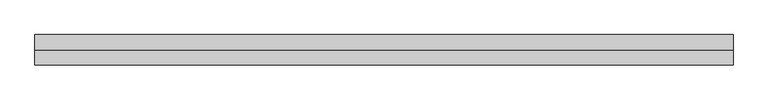
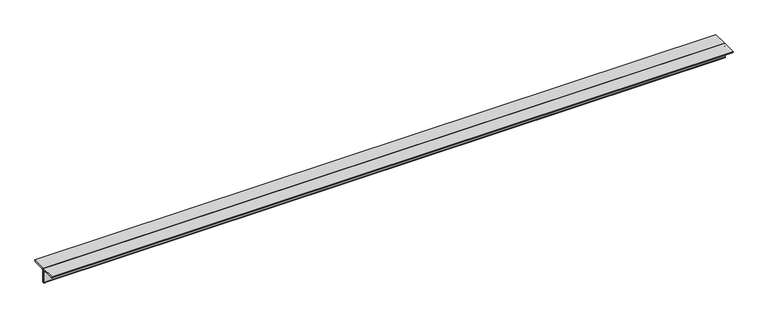
"""IFC4 building model written with IfcOpenShell, lengths in millimetres: member geometry, 0123_Steel Framing_2Ls-KSD3502 : H_SB_AR_S03_2Ls-130x130x12_HBR1."""

import ifcopenshell
import ifcopenshell.guid

model = None  # the IFC model being written
_history = None  # IfcOwnerHistory: only IFC2X3 demands one
_inside = {}  # id of a spatial element -> (the spatial element, [elements in it])
_under = {}  # id of a project, library or spatial element -> (it, [spatial elements below it])
_declared = {}  # id of a project -> (the project, [libraries it declares])
_typed = {}  # id of a type object -> (the type object, [elements of that type])
_made_of = {}  # id of a material, layer set ... -> (it, [elements and type objects made of it])


def new_model(schema):
    """Start an empty IFC model of exactly this schema.

    Asked for "IFC4X3", IfcOpenShell would pick the latest addendum, in which some entities
    have other attributes; the version numbers below select the first issue.
    IFC2X3 requires an IfcOwnerHistory on every rooted entity: one is made here for all.
    """
    global model, _history
    if schema == "IFC4X3":
        model = ifcopenshell.file(schema_version=(4, 3, 0, 0))
    else:
        model = ifcopenshell.file(schema=schema)
    _inside.clear()
    _under.clear()
    _declared.clear()
    _typed.clear()
    _made_of.clear()
    _history = None
    if model.schema == "IFC2X3":
        org = make("IfcOrganization", Name="unknown")
        user = make(
            "IfcPersonAndOrganization",
            ThePerson=make("IfcPerson", FamilyName="unknown"),
            TheOrganization=org,
        )
        app = make(
            "IfcApplication",
            ApplicationDeveloper=org,
            Version="unknown",
            ApplicationFullName="unknown",
            ApplicationIdentifier="unknown",
        )
        _history = make(
            "IfcOwnerHistory",
            OwningUser=user,
            OwningApplication=app,
            ChangeAction="ADDED",
            CreationDate=0,
        )
    return model


def make(cls, **values):
    """One entity of the class cls with the attributes given. An attribute that is None is left unset."""
    return model.create_entity(
        cls, **{name: value for name, value in values.items() if value is not None}
    )


def rooted(cls, **values):
    """An entity with a GlobalId (a new one), such as an element, a storey or a relation."""
    return make(cls, GlobalId=ifcopenshell.guid.new(), OwnerHistory=_history, **values)


def si_unit(unit_type, name, prefix=None):
    """IfcSIUnit, for example si_unit("LENGTHUNIT", "METRE", prefix="MILLI")."""
    return make("IfcSIUnit", UnitType=unit_type, Prefix=prefix, Name=name)


def assignment(units):
    """IfcUnitAssignment: the units of a project."""
    return None if units is None else make("IfcUnitAssignment", Units=units)


def point(xyz):
    """IfcCartesianPoint."""
    return None if xyz is None else make("IfcCartesianPoint", Coordinates=xyz)


def direction(xyz):
    """IfcDirection."""
    return None if xyz is None else make("IfcDirection", DirectionRatios=xyz)


def frame(location, z_axis=None, x_axis=None):
    """IfcAxis2Placement3D, a coordinate frame: its origin and axes. An axis left out is left unset."""
    return make(
        "IfcAxis2Placement3D",
        Location=point(location),
        Axis=direction(z_axis),
        RefDirection=direction(x_axis),
    )


def frame_2d(location, x_axis=None):
    """IfcAxis2Placement2D, a coordinate frame in the plane: its origin and x axis."""
    return make(
        "IfcAxis2Placement2D", Location=point(location), RefDirection=direction(x_axis)
    )


def origin():
    """The frame at (0, 0, 0) with its axes left unset."""
    return frame((0.0, 0.0, 0.0))


def place(relative_to, where):
    """IfcLocalPlacement: puts the frame where relative to a parent placement (None: the world)."""
    return make(
        "IfcLocalPlacement", PlacementRelTo=relative_to, RelativePlacement=where
    )


def context(
    kind, dimensions, precision=None, world=None, true_north=None, identifier=None
):
    """IfcGeometricRepresentationContext, for example the 3D "Model" context."""
    return make(
        "IfcGeometricRepresentationContext",
        ContextIdentifier=identifier,
        ContextType=kind,
        CoordinateSpaceDimension=dimensions,
        Precision=precision,
        WorldCoordinateSystem=world,
        TrueNorth=true_north,
    )


def project(units=None, contexts=None):
    """IfcProject with its units and contexts."""
    return rooted(
        "IfcProject",
        Name="project",
        RepresentationContexts=contexts,
        UnitsInContext=assignment(units),
    )


def spatial(cls, under=None, at=None, **own):
    """A site, building, storey or space (cls), placed at a placement, below another one or the project."""
    s = rooted(cls, ObjectPlacement=at, **own)
    if under is not None:
        _under.setdefault(under.id(), (under, []))[1].append(s)
    return s


def polyline(points):
    """IfcPolyline through the points."""
    return make("IfcPolyline", Points=[point(p) for p in points])


def circle_curve(where, radius):
    """IfcCircle in the frame where."""
    return make("IfcCircle", Position=where, Radius=radius)


def trimmed(basis, trim1, trim2, sense, master):
    """IfcTrimmedCurve: the piece of a basis curve between two trims."""
    return make(
        "IfcTrimmedCurve",
        BasisCurve=basis,
        Trim1=trim1,
        Trim2=trim2,
        SenseAgreement=sense,
        MasterRepresentation=master,
    )


def segment(curve, same_sense, transition):
    """IfcCompositeCurveSegment."""
    return make(
        "IfcCompositeCurveSegment",
        Transition=transition,
        SameSense=same_sense,
        ParentCurve=curve,
    )


def composite_curve(segments, self_intersect=None):
    """IfcCompositeCurve: segments joined end to end."""
    return make("IfcCompositeCurve", Segments=segments, SelfIntersect=self_intersect)


def outline(outer, holes=None, kind="AREA"):
    """IfcArbitraryClosedProfileDef: a profile drawn as a closed curve; with holes, ...WithVoids."""
    if holes is None:
        return make("IfcArbitraryClosedProfileDef", ProfileType=kind, OuterCurve=outer)
    return make(
        "IfcArbitraryProfileDefWithVoids",
        ProfileType=kind,
        OuterCurve=outer,
        InnerCurves=holes,
    )


def extrude(swept, where, along, depth):
    """IfcExtrudedAreaSolid: the profile swept, set in the frame where, extruded along a direction by depth."""
    return make(
        "IfcExtrudedAreaSolid",
        SweptArea=swept,
        Position=where,
        ExtrudedDirection=direction(along),
        Depth=depth,
    )


def shape(context_of_items, identifier, shape_type, items):
    """IfcShapeRepresentation: the items that make up one representation, for example the "Body"."""
    return make(
        "IfcShapeRepresentation",
        ContextOfItems=context_of_items,
        RepresentationIdentifier=identifier,
        RepresentationType=shape_type,
        Items=items,
    )


def source(mapping_origin, context_of_items, identifier, shape_type, items):
    """IfcRepresentationMap: a shape defined once, which mapped items show again and again."""
    return make(
        "IfcRepresentationMap",
        MappingOrigin=mapping_origin,
        MappedRepresentation=shape(context_of_items, identifier, shape_type, items),
    )


def transform(
    local_origin,
    x_axis=None,
    y_axis=None,
    z_axis=None,
    scale=None,
    scale2=None,
    scale3=None,
    uniform=True,
):
    """IfcCartesianTransformationOperator3D, or its non-uniform kind. x_axis, y_axis, z_axis: its Axis1, 2, 3."""
    if uniform:
        return make(
            "IfcCartesianTransformationOperator3D",
            Axis1=direction(x_axis),
            Axis2=direction(y_axis),
            LocalOrigin=point(local_origin),
            Scale=scale,
            Axis3=direction(z_axis),
        )
    return make(
        "IfcCartesianTransformationOperator3DnonUniform",
        Axis1=direction(x_axis),
        Axis2=direction(y_axis),
        LocalOrigin=point(local_origin),
        Scale=scale,
        Axis3=direction(z_axis),
        Scale2=scale2,
        Scale3=scale3,
    )


def mapped(mapping_source, mapping_target):
    """IfcMappedItem: shows the shape of a source again, moved by a transform."""
    return make(
        "IfcMappedItem", MappingSource=mapping_source, MappingTarget=mapping_target
    )


def made_of(thing, what):
    """Note that an element or type object is made of a material, layer set ...; save() writes the relation."""
    if what is not None:
        _made_of.setdefault(what.id(), (what, []))[1].append(thing)
    return thing


def element(
    cls,
    number,
    at=None,
    inside=None,
    cuts=None,
    type_object=None,
    material=None,
    context=None,
    identifier="Body",
    shape_type=None,
    held_by="IfcProductDefinitionShape",
    body=None,
    shapes=None,
    **own,
):
    """One element of the class cls, such as IfcWall. Its Tag is "e" and its number.

    at: its placement. inside: the storey or other place that contains it. cuts: it is an
    opening in that element (IfcRelVoidsElement). A single representation is given by context,
    identifier, shape_type and body (its items); several are given by shapes. held_by: the class
    of the entity that holds the representations. save() writes the other relations.
    """
    e = rooted(cls, Tag="e%d" % number, ObjectPlacement=at, **own)
    if body is not None:
        shapes = [shape(context, identifier, shape_type, body)]
    if shapes is not None:
        e.Representation = make(held_by, Representations=shapes)
    if inside is not None:
        _inside.setdefault(inside.id(), (inside, []))[1].append(e)
    if cuts is not None:
        rooted(
            "IfcRelVoidsElement", RelatingBuildingElement=cuts, RelatedOpeningElement=e
        )
    if type_object is not None:
        _typed.setdefault(type_object.id(), (type_object, []))[1].append(e)
    return made_of(e, material)


def aggregate(whole, parts):
    """IfcRelAggregates: a whole, such as a stair, and the parts it consists of."""
    return rooted("IfcRelAggregates", RelatingObject=whole, RelatedObjects=parts)


def save(model, path):
    """Write the relations noted so far, then the file.

    IfcRelAggregates (storeys below a building ...), IfcRelContainedInSpatialStructure (elements
    in a storey), IfcRelDefinesByType, IfcRelAssociatesMaterial and IfcRelDeclares: one each for
    every whole, place, type object, material and project.
    """
    for whole, parts in _under.values():
        aggregate(whole, parts)
    for where, things in _inside.values():
        rooted(
            "IfcRelContainedInSpatialStructure",
            RelatedElements=things,
            RelatingStructure=where,
        )
    for kind, things in _typed.values():
        rooted("IfcRelDefinesByType", RelatedObjects=things, RelatingType=kind)
    for what, things in _made_of.values():
        rooted("IfcRelAssociatesMaterial", RelatedObjects=things, RelatingMaterial=what)
    for by, libraries in _declared.values():
        rooted("IfcRelDeclares", RelatingContext=by, RelatedDefinitions=libraries)
    model.write(path)


def member_93b6b39c(model_context):
    return source(origin(), model_context, "Body", "SweptSolid", [
        extrude(outline(composite_curve([segment(polyline([(0.0, 36.4), (130.0, 36.4)]), True, "CONTINUOUS"), segment(trimmed(circle_curve(frame_2d((118.0, 36.4)), 12.0), [point((130.0, 36.4))], [point((118.0, 24.4))], False, "CARTESIAN"), True, "CONTINUOUS"), segment(polyline([(118.0, 24.4), (24.0, 24.4)]), True, "CONTINUOUS"), segment(trimmed(circle_curve(frame_2d((24.0, 12.4)), 12.0), [point((24.0, 24.4))], [point((12.0, 12.4))], True, "CARTESIAN"), True, "CONTINUOUS"), segment(polyline([(12.0, 12.4), (12.0, -81.6)]), True, "CONTINUOUS"), segment(trimmed(circle_curve(frame_2d((0.0, -81.6)), 12.0), [point((12.0, -81.6))], [point((0.0, -93.6))], False, "CARTESIAN"), True, "CONTINUOUS"), segment(polyline([(0.0, -93.6), (0.0, 36.4)]), True, "CONTINUOUS")], self_intersect=False)), frame((-2923.1123523, 0.0, 0.0), z_axis=(1.0, 0.0, 0.0), x_axis=(0.0, 1.0, 0.0)), (0.0, 0.0, 1.0), 5953.2348533),
        extrude(outline(composite_curve([segment(polyline([(0.0, 36.4), (0.0, -93.6)]), True, "CONTINUOUS"), segment(trimmed(circle_curve(frame_2d((0.0, -81.6)), 12.0), [point((0.0, -93.6))], [point((-12.0, -81.6))], False, "CARTESIAN"), True, "CONTINUOUS"), segment(polyline([(-12.0, -81.6), (-12.0, 12.4)]), True, "CONTINUOUS"), segment(trimmed(circle_curve(frame_2d((-24.0, 12.4)), 12.0), [point((-12.0, 12.4))], [point((-24.0, 24.4))], True, "CARTESIAN"), True, "CONTINUOUS"), segment(polyline([(-24.0, 24.4), (-118.0, 24.4)]), True, "CONTINUOUS"), segment(trimmed(circle_curve(frame_2d((-118.0, 36.4)), 12.0), [point((-118.0, 24.4))], [point((-130.0, 36.4))], False, "CARTESIAN"), True, "CONTINUOUS"), segment(polyline([(-130.0, 36.4), (0.0, 36.4)]), True, "CONTINUOUS")], self_intersect=False)), frame((-2923.1123523, 0.0, 0.0), z_axis=(1.0, 0.0, 0.0), x_axis=(0.0, 1.0, 0.0)), (0.0, 0.0, 1.0), 5953.2348533),
    ])


if __name__ == "__main__":
    model = new_model("IFC4")
    model_context = context("Model", 3, world=origin())
    ifc_project = project(units=[si_unit("LENGTHUNIT", "METRE", prefix="MILLI")], contexts=[model_context])
    site = spatial("IfcSite", under=ifc_project)
    building = spatial("IfcBuilding", under=site)
    placement = place(None, origin())
    member_shape = member_93b6b39c(model_context)
    element("IfcMember", 1, ObjectType="0123_Steel Framing_2Ls-KSD3502 : H_SB_AR_S03_2Ls-130x130x12_HBR1", at=placement, inside=building, context=model_context, shape_type="MappedRepresentation", body=[
        mapped(member_shape, transform((0.0, 0.0, 0.0), x_axis=(1.0, 0.0, 0.0), y_axis=(0.0, 1.0, 0.0), z_axis=(0.0, 0.0, 1.0))),
    ])
    save(model, "model.ifc")

# Revit data of these elements
# Type "0123_Steel Framing_2Ls-KSD3502 : H_SB_AR_S03_2Ls-130x130x12_HBR1"
#   Assembly Code = "B10"
#   Legs = "SLBB"
#   W = 8.97
#   Perimeter = 1.04 m²/m
#   Nominal Weight = 46.80 kgf/m
#   Length [instance default] = 1000 mm
#   Space = 0 mm
#   b = 130 mm
#   d = 130 mm
#   t = 12 mm
#   y = 36.4 mm
#   A = 0.005952 m²
#   Structural Material [instance default] = Steel ASTM A36
# Element 1 (IfcMember, "0123_Steel Framing_2Ls-KSD3502 : H_SB_AR_S03_2Ls-130x130x12_HBR1")
#   Structural Material = Steel, 45-345
#   Materials on its faces: "Steel, 45-345"
# Materials
#   "Steel ASTM A36": class "Metal", colour RGB 199 199 199, transparency 0, Description = "Structural steel, ASTM A36 Grade B, mill finish", Cost = 0
#   "Steel, 45-345": class "Metal", colour RGB 189 187 185, transparency 0, Description = "Steel 345 MPa", Cost = 0
